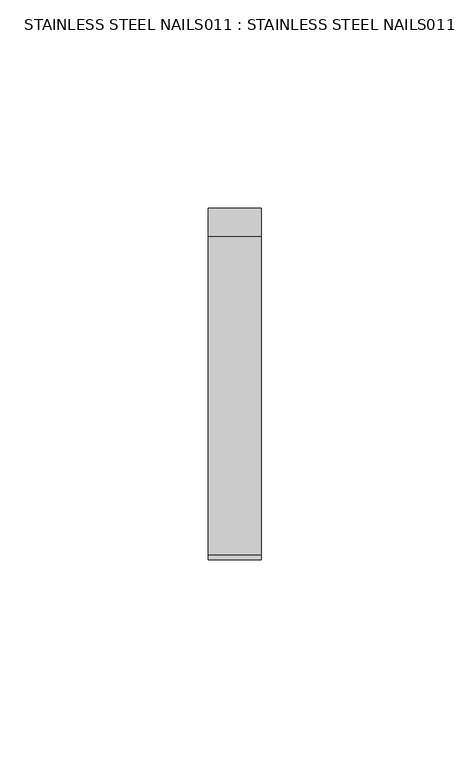
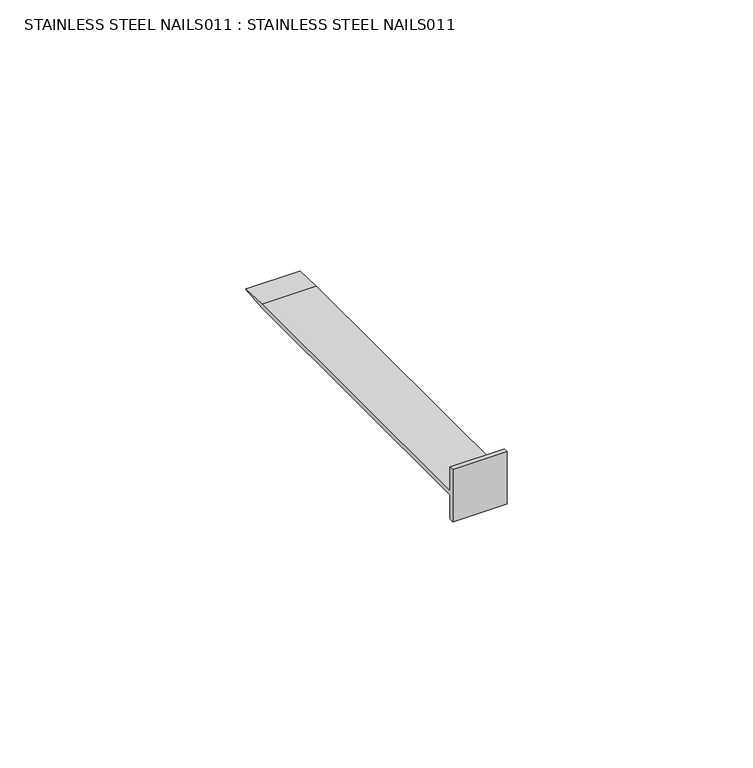
"""IFC4 building model written with IfcOpenShell, lengths in millimetres: proxy geometry, STAINLESS STEEL NAILS011 : STAINLESS STEEL NAILS011."""

import ifcopenshell
import ifcopenshell.guid

model = None  # the IFC model being written
_history = None  # IfcOwnerHistory: only IFC2X3 demands one
_inside = {}  # id of a spatial element -> (the spatial element, [elements in it])
_under = {}  # id of a project, library or spatial element -> (it, [spatial elements below it])
_declared = {}  # id of a project -> (the project, [libraries it declares])
_typed = {}  # id of a type object -> (the type object, [elements of that type])
_made_of = {}  # id of a material, layer set ... -> (it, [elements and type objects made of it])


def new_model(schema):
    """Start an empty IFC model of exactly this schema.

    Asked for "IFC4X3", IfcOpenShell would pick the latest addendum, in which some entities
    have other attributes; the version numbers below select the first issue.
    IFC2X3 requires an IfcOwnerHistory on every rooted entity: one is made here for all.
    """
    global model, _history
    if schema == "IFC4X3":
        model = ifcopenshell.file(schema_version=(4, 3, 0, 0))
    else:
        model = ifcopenshell.file(schema=schema)
    _inside.clear()
    _under.clear()
    _declared.clear()
    _typed.clear()
    _made_of.clear()
    _history = None
    if model.schema == "IFC2X3":
        org = make("IfcOrganization", Name="unknown")
        user = make(
            "IfcPersonAndOrganization",
            ThePerson=make("IfcPerson", FamilyName="unknown"),
            TheOrganization=org,
        )
        app = make(
            "IfcApplication",
            ApplicationDeveloper=org,
            Version="unknown",
            ApplicationFullName="unknown",
            ApplicationIdentifier="unknown",
        )
        _history = make(
            "IfcOwnerHistory",
            OwningUser=user,
            OwningApplication=app,
            ChangeAction="ADDED",
            CreationDate=0,
        )
    return model


def make(cls, **values):
    """One entity of the class cls with the attributes given. An attribute that is None is left unset."""
    return model.create_entity(
        cls, **{name: value for name, value in values.items() if value is not None}
    )


def rooted(cls, **values):
    """An entity with a GlobalId (a new one), such as an element, a storey or a relation."""
    return make(cls, GlobalId=ifcopenshell.guid.new(), OwnerHistory=_history, **values)


def si_unit(unit_type, name, prefix=None):
    """IfcSIUnit, for example si_unit("LENGTHUNIT", "METRE", prefix="MILLI")."""
    return make("IfcSIUnit", UnitType=unit_type, Prefix=prefix, Name=name)


def assignment(units):
    """IfcUnitAssignment: the units of a project."""
    return None if units is None else make("IfcUnitAssignment", Units=units)


def point(xyz):
    """IfcCartesianPoint."""
    return None if xyz is None else make("IfcCartesianPoint", Coordinates=xyz)


def direction(xyz):
    """IfcDirection."""
    return None if xyz is None else make("IfcDirection", DirectionRatios=xyz)


def frame(location, z_axis=None, x_axis=None):
    """IfcAxis2Placement3D, a coordinate frame: its origin and axes. An axis left out is left unset."""
    return make(
        "IfcAxis2Placement3D",
        Location=point(location),
        Axis=direction(z_axis),
        RefDirection=direction(x_axis),
    )


def origin():
    """The frame at (0, 0, 0) with its axes left unset."""
    return frame((0.0, 0.0, 0.0))


def place(relative_to, where):
    """IfcLocalPlacement: puts the frame where relative to a parent placement (None: the world)."""
    return make(
        "IfcLocalPlacement", PlacementRelTo=relative_to, RelativePlacement=where
    )


def context(
    kind, dimensions, precision=None, world=None, true_north=None, identifier=None
):
    """IfcGeometricRepresentationContext, for example the 3D "Model" context."""
    return make(
        "IfcGeometricRepresentationContext",
        ContextIdentifier=identifier,
        ContextType=kind,
        CoordinateSpaceDimension=dimensions,
        Precision=precision,
        WorldCoordinateSystem=world,
        TrueNorth=true_north,
    )


def project(units=None, contexts=None):
    """IfcProject with its units and contexts."""
    return rooted(
        "IfcProject",
        Name="project",
        RepresentationContexts=contexts,
        UnitsInContext=assignment(units),
    )


def spatial(cls, under=None, at=None, **own):
    """A site, building, storey or space (cls), placed at a placement, below another one or the project."""
    s = rooted(cls, ObjectPlacement=at, **own)
    if under is not None:
        _under.setdefault(under.id(), (under, []))[1].append(s)
    return s


def polyline(points):
    """IfcPolyline through the points."""
    return make("IfcPolyline", Points=[point(p) for p in points])


def outline(outer, holes=None, kind="AREA"):
    """IfcArbitraryClosedProfileDef: a profile drawn as a closed curve; with holes, ...WithVoids."""
    if holes is None:
        return make("IfcArbitraryClosedProfileDef", ProfileType=kind, OuterCurve=outer)
    return make(
        "IfcArbitraryProfileDefWithVoids",
        ProfileType=kind,
        OuterCurve=outer,
        InnerCurves=holes,
    )


def extrude(swept, where, along, depth):
    """IfcExtrudedAreaSolid: the profile swept, set in the frame where, extruded along a direction by depth."""
    return make(
        "IfcExtrudedAreaSolid",
        SweptArea=swept,
        Position=where,
        ExtrudedDirection=direction(along),
        Depth=depth,
    )


def shape(context_of_items, identifier, shape_type, items):
    """IfcShapeRepresentation: the items that make up one representation, for example the "Body"."""
    return make(
        "IfcShapeRepresentation",
        ContextOfItems=context_of_items,
        RepresentationIdentifier=identifier,
        RepresentationType=shape_type,
        Items=items,
    )


def source(mapping_origin, context_of_items, identifier, shape_type, items):
    """IfcRepresentationMap: a shape defined once, which mapped items show again and again."""
    return make(
        "IfcRepresentationMap",
        MappingOrigin=mapping_origin,
        MappedRepresentation=shape(context_of_items, identifier, shape_type, items),
    )


def transform(
    local_origin,
    x_axis=None,
    y_axis=None,
    z_axis=None,
    scale=None,
    scale2=None,
    scale3=None,
    uniform=True,
):
    """IfcCartesianTransformationOperator3D, or its non-uniform kind. x_axis, y_axis, z_axis: its Axis1, 2, 3."""
    if uniform:
        return make(
            "IfcCartesianTransformationOperator3D",
            Axis1=direction(x_axis),
            Axis2=direction(y_axis),
            LocalOrigin=point(local_origin),
            Scale=scale,
            Axis3=direction(z_axis),
        )
    return make(
        "IfcCartesianTransformationOperator3DnonUniform",
        Axis1=direction(x_axis),
        Axis2=direction(y_axis),
        LocalOrigin=point(local_origin),
        Scale=scale,
        Axis3=direction(z_axis),
        Scale2=scale2,
        Scale3=scale3,
    )


def mapped(mapping_source, mapping_target):
    """IfcMappedItem: shows the shape of a source again, moved by a transform."""
    return make(
        "IfcMappedItem", MappingSource=mapping_source, MappingTarget=mapping_target
    )


def made_of(thing, what):
    """Note that an element or type object is made of a material, layer set ...; save() writes the relation."""
    if what is not None:
        _made_of.setdefault(what.id(), (what, []))[1].append(thing)
    return thing


def element(
    cls,
    number,
    at=None,
    inside=None,
    cuts=None,
    type_object=None,
    material=None,
    context=None,
    identifier="Body",
    shape_type=None,
    held_by="IfcProductDefinitionShape",
    body=None,
    shapes=None,
    **own,
):
    """One element of the class cls, such as IfcWall. Its Tag is "e" and its number.

    at: its placement. inside: the storey or other place that contains it. cuts: it is an
    opening in that element (IfcRelVoidsElement). A single representation is given by context,
    identifier, shape_type and body (its items); several are given by shapes. held_by: the class
    of the entity that holds the representations. save() writes the other relations.
    """
    e = rooted(cls, Tag="e%d" % number, ObjectPlacement=at, **own)
    if body is not None:
        shapes = [shape(context, identifier, shape_type, body)]
    if shapes is not None:
        e.Representation = make(held_by, Representations=shapes)
    if inside is not None:
        _inside.setdefault(inside.id(), (inside, []))[1].append(e)
    if cuts is not None:
        rooted(
            "IfcRelVoidsElement", RelatingBuildingElement=cuts, RelatedOpeningElement=e
        )
    if type_object is not None:
        _typed.setdefault(type_object.id(), (type_object, []))[1].append(e)
    return made_of(e, material)


def aggregate(whole, parts):
    """IfcRelAggregates: a whole, such as a stair, and the parts it consists of."""
    return rooted("IfcRelAggregates", RelatingObject=whole, RelatedObjects=parts)


def save(model, path):
    """Write the relations noted so far, then the file.

    IfcRelAggregates (storeys below a building ...), IfcRelContainedInSpatialStructure (elements
    in a storey), IfcRelDefinesByType, IfcRelAssociatesMaterial and IfcRelDeclares: one each for
    every whole, place, type object, material and project.
    """
    for whole, parts in _under.values():
        aggregate(whole, parts)
    for where, things in _inside.values():
        rooted(
            "IfcRelContainedInSpatialStructure",
            RelatedElements=things,
            RelatingStructure=where,
        )
    for kind, things in _typed.values():
        rooted("IfcRelDefinesByType", RelatedObjects=things, RelatingType=kind)
    for what, things in _made_of.values():
        rooted("IfcRelAssociatesMaterial", RelatedObjects=things, RelatingMaterial=what)
    for by, libraries in _declared.values():
        rooted("IfcRelDeclares", RelatingContext=by, RelatedDefinitions=libraries)
    model.write(path)


def stainless_steel_nails011_stainless_steel_nails011_743e7744(model_context):
    return source(origin(), model_context, "Body", "SweptSolid", [
        extrude(outline(polyline([(-5577.1765463, 40184.7938624), (-5577.1765463, 40197.7922463), (-5576.0933476, 40197.7922463), (-5576.0933476, 40191.8346536), (-5499.5272732, 40191.8346536), (-5492.898107, 40191.472848), (-5499.5272732, 40190.751455), (-5576.0933476, 40190.751455), (-5576.0933476, 40184.7938624), (-5577.1765463, 40184.7938624)])), frame((14383.0178845, 0.0, 0.0), z_axis=(1.0, 0.0, 0.0), x_axis=(0.0, 1.0, 0.0)), (0.0, 0.0, 1.0), 12.7),
    ])


if __name__ == "__main__":
    model = new_model("IFC4")
    model_context = context("Model", 3, world=origin())
    ifc_project = project(units=[si_unit("LENGTHUNIT", "METRE", prefix="MILLI")], contexts=[model_context])
    site = spatial("IfcSite", under=ifc_project)
    building = spatial("IfcBuilding", under=site)
    placement = place(None, origin())
    stainless_steel_nails011_stainless_steel_nails011_shape = stainless_steel_nails011_stainless_steel_nails011_743e7744(model_context)
    element("IfcBuildingElementProxy", 1, Name="STAINLESS STEEL NAILS011 : STAINLESS STEEL NAILS011", ObjectType="STAINLESS STEEL NAILS011 : STAINLESS STEEL NAILS011", at=placement, inside=building, context=model_context, shape_type="MappedRepresentation", body=[
        mapped(stainless_steel_nails011_stainless_steel_nails011_shape, transform((0.0, 0.0, 0.0), x_axis=(1.0, 0.0, 0.0), y_axis=(0.0, 1.0, 0.0), z_axis=(0.0, 0.0, 1.0))),
    ])
    save(model, "model.ifc")

# Revit data of these elements
# Type "STAINLESS STEEL NAILS011 : STAINLESS STEEL NAILS011"
#   NameOverride = "STAINLESS STEEL NAILS011"
# Element 1 (IfcBuildingElementProxy, "STAINLESS STEEL NAILS011 : STAINLESS STEEL NAILS011")
#   Materials on its faces: "1 3/4\" STAINLESS STEEL RINGSHANK 5D COMMON NAILS @ 4\" (101.6MM) O.C. FIRESTONE PROVIDED MAX., 1/2\" STAGGERED"
# Materials
#   "1 3/4\" STAINLESS STEEL RINGSHANK 5D COMMON NAILS @ 4\" (101.6MM) O.C. FIRESTONE PROVIDED MAX., 1/2\" STAGGERED": class "Unassigned", colour RGB 255 255 255, transparency 0
